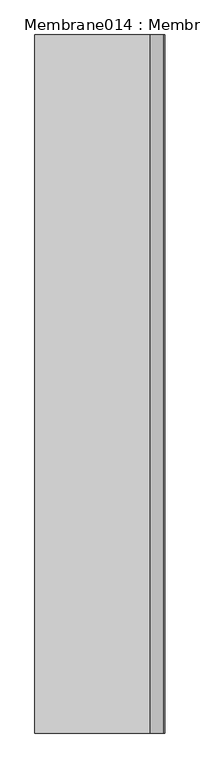
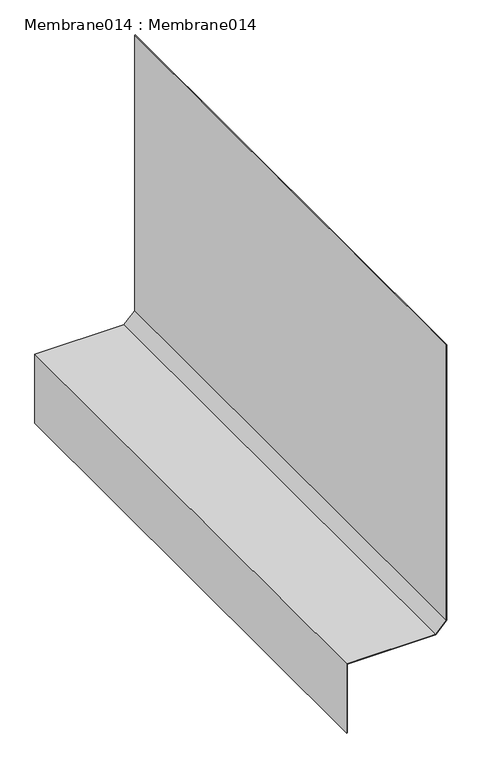
"""IFC4 building model written with IfcOpenShell, lengths in millimetres: proxy geometry, Membrane014 : Membrane014."""

from ifc_helpers import new_model, si_unit, frame, origin, place, context, project, spatial, polyline, outline, extrude, source, transform, mapped, element, save


def membrane014_membrane014_7a283e70(model_context):
    return source(origin(), model_context, "Body", "SweptSolid", [
        extrude(outline(polyline([(33706.6732458, -9663.9882813), (32626.9430944, -9663.9882813), (32586.6386719, -9703.8524464), (32586.6386719, -10033.7987014), (32314.8961275, -10033.7987014), (32314.8961275, -10031.7987014), (32584.6386719, -10031.7987014), (32584.6386719, -9703.0175781), (32626.1210938, -9661.9882813), (33706.6732458, -9661.9882813), (33706.6732458, -9663.9882813)])), frame((0.0, 7182.1531721, 0.0), z_axis=(0.0, 1.0, 0.0), x_axis=(0.0, 0.0, 1.0)), (0.0, 0.0, 1.0), 2000.0),
    ])


if __name__ == "__main__":
    model = new_model("IFC4")
    model_context = context("Model", 3, world=origin())
    ifc_project = project(units=[si_unit("LENGTHUNIT", "METRE", prefix="MILLI")], contexts=[model_context])
    site = spatial("IfcSite", under=ifc_project)
    building = spatial("IfcBuilding", under=site)
    placement = place(None, origin())
    membrane014_membrane014_shape = membrane014_membrane014_7a283e70(model_context)
    element("IfcBuildingElementProxy", 1, Name="Membrane014 : Membrane014", ObjectType="Membrane014 : Membrane014", at=placement, inside=building, context=model_context, shape_type="MappedRepresentation", body=[
        mapped(membrane014_membrane014_shape, transform((0.0, 0.0, 0.0), x_axis=(1.0, 0.0, 0.0), y_axis=(0.0, 1.0, 0.0), z_axis=(0.0, 0.0, 1.0))),
    ])
    save(model, "model.ifc")

# Revit data of these elements
# Type "Membrane014 : Membrane014"
#   NameOverride = "Membrane014"
# Element 1 (IfcBuildingElementProxy, "Membrane014 : Membrane014")
#   Materials on its faces: "BITUMINOUS MEMBRANE"
# Materials
#   "BITUMINOUS MEMBRANE": class "Unassigned", colour RGB 0 171 31, transparency 0, Cost = 0
